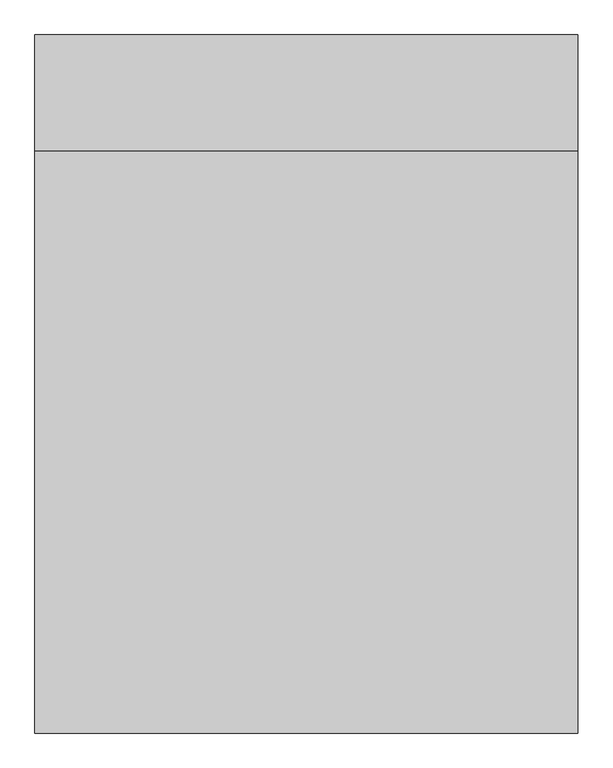
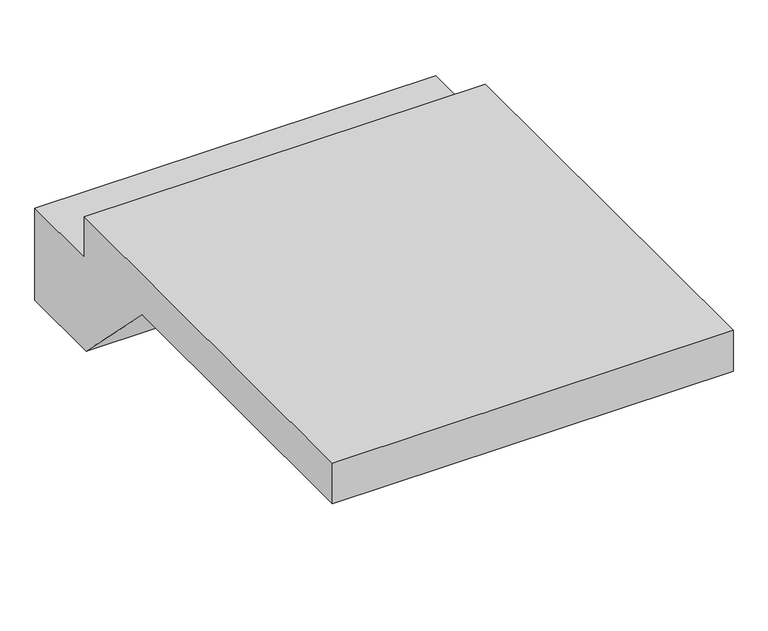
"""IFC4 building model written with IfcOpenShell, lengths in millimetres: proxy geometry, 벽 1 : 벽 1."""

from ifc_helpers import new_model, si_unit, frame, origin, place, context, project, spatial, polyline, outline, extrude, source, transform, mapped, element, save


def generic_models_c40cd3bd(model_context):
    return source(origin(), model_context, "Body", "SweptSolid", [
        extrude(outline(polyline([(40819.5208589, 599.905241), (40819.5208589, 449.905241), (41119.5208589, 449.905241), (41119.5208589, 109.2314637), (40810.1946362, 109.2314637), (40469.5208589, 449.905241), (39319.5208589, 449.905241), (39319.5208589, 599.905241), (40819.5208589, 599.905241)])), frame((21000.0, 0.0, 0.0), z_axis=(1.0, 0.0, 0.0), x_axis=(0.0, 1.0, 0.0)), (0.0, 0.0, 1.0), 1400.0),
    ])


if __name__ == "__main__":
    model = new_model("IFC4")
    model_context = context("Model", 3, world=origin())
    ifc_project = project(units=[si_unit("LENGTHUNIT", "METRE", prefix="MILLI")], contexts=[model_context])
    site = spatial("IfcSite", under=ifc_project)
    building = spatial("IfcBuilding", under=site)
    placement = place(None, origin())
    generic_models_shape = generic_models_c40cd3bd(model_context)
    element("IfcBuildingElementProxy", 1, Name="벽 1 : 벽 1", ObjectType="벽 1 : 벽 1", at=placement, inside=building, context=model_context, shape_type="MappedRepresentation", body=[
        mapped(generic_models_shape, transform((0.0, 0.0, 0.0), x_axis=(1.0, 0.0, 0.0), y_axis=(0.0, 1.0, 0.0), z_axis=(0.0, 0.0, 1.0))),
    ])
    save(model, "model.ifc")

# Revit data of these elements
# Element 1 (IfcBuildingElementProxy, "벽 1 : 벽 1")
#   Materials on its faces: "A03AC032-00007_Structural Concrete_Type1_25MPa-30Mpa"
# Materials
#   "A03AC032-00007_Structural Concrete_Type1_25MPa-30Mpa": class "Concrete", colour RGB 176 176 176, transparency 0, Keynote = "09910.A1", Description = "Reinf. Conc.", W00) Work Master Code = "A03AC032-00007", W01) Work Master_Lv1 = "Concrete Work", W02) Work Master_Lv2 = "Substructure Work", W03) Work Master_Spec.1 = "Structural Concrete", W04) Work Master_Spec.2 = "Cement Type-1", W05) Work Master_Spec.3 = "25MPa < F'c (Cylinder Strength) ≤ 30MPa", Cost = 0
